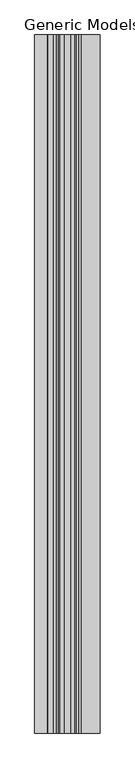
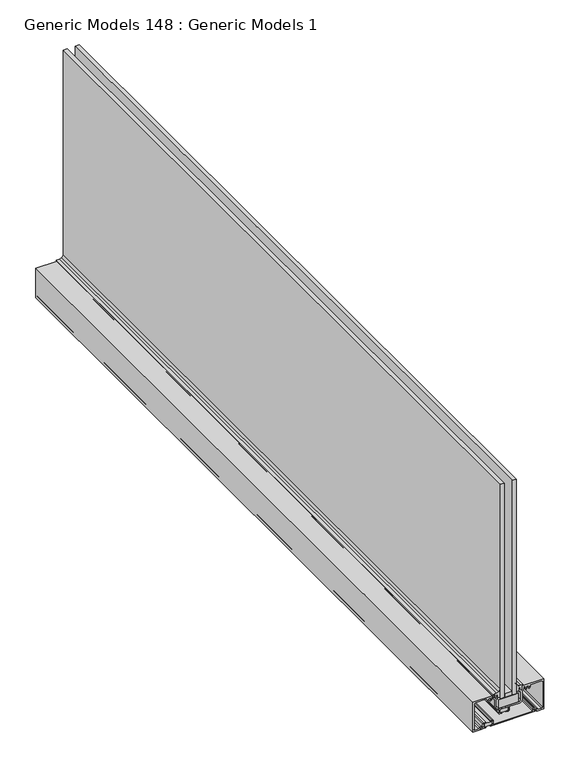
"""IFC4 building model written with IfcOpenShell, lengths in millimetres: proxy geometry, Generic Models 148 : Generic Models 1."""

from ifc_helpers import new_model, si_unit, point, frame, frame_2d, origin, place, context, project, spatial, polyline, circle_curve, trimmed, segment, composite_curve, outline, extrude, source, transform, mapped, element, save


def generic_models_148_generic_models_1_cbf84703(model_context):
    return source(origin(), model_context, "Body", "SweptSolid", [
        extrude(outline(composite_curve([segment(trimmed(circle_curve(frame_2d((-1910.3503206, 53784.0362451)), 1.5795625), [point((-1908.7707581, 53784.0362451))], [point((-1909.8092658, 53782.5522379))], False, "CARTESIAN"), True, "CONTINUOUS"), segment(polyline([(-1909.8092658, 53782.5522379), (-1913.6824831, 53781.1401001), (-1913.6824831, 53782.6297743), (-1916.2637581, 53782.6297743), (-1916.2637581, 53778.3117743), (-1917.8988831, 53778.3117743), (-1917.8988831, 53787.5924263), (-1916.2637581, 53787.5924263), (-1916.2637581, 53784.0110263), (-1909.6438831, 53784.0110263), (-1909.6438831, 53787.5924263), (-1908.7707581, 53787.5924263), (-1908.7707581, 53784.0362451)]), True, "CONTINUOUS")], self_intersect=False)), frame((0.0, 0.0, 0.0), z_axis=(0.0, 1.0, 0.0), x_axis=(0.0, 0.0, 1.0)), (0.0, 0.0, 1.0), 1219.2),
        extrude(outline(composite_curve([segment(trimmed(circle_curve(frame_2d((-1912.0013206, 53863.1457105)), 0.7064375), [point((-1911.7594231, 53863.809442))], [point((-1912.7064566, 53863.102848))], True, "CARTESIAN"), True, "CONTINUOUS"), segment(polyline([(-1912.7064566, 53863.102848), (-1916.2637581, 53863.102848), (-1916.2637581, 53800.0082638)]), True, "CONTINUOUS"), segment(trimmed(circle_curve(frame_2d((-1915.5573206, 53800.0082638)), 0.7064375), [point((-1916.2637581, 53800.0082638))], [point((-1915.5573206, 53799.3018263))], True, "CARTESIAN"), True, "CONTINUOUS"), segment(polyline([(-1915.5573206, 53799.3018263), (-1910.3503206, 53799.3018263)]), True, "CONTINUOUS"), segment(trimmed(circle_curve(frame_2d((-1910.3503206, 53797.7222638)), 1.5795625), [point((-1910.3503206, 53799.3018263))], [point((-1908.7707581, 53797.7222638))], False, "CARTESIAN"), True, "CONTINUOUS"), segment(polyline([(-1908.7707581, 53797.7222638), (-1908.7707581, 53794.3393013), (-1909.6438831, 53794.3393013), (-1909.6438831, 53797.9207013), (-1916.2637581, 53797.9207013), (-1916.2637581, 53794.3393013), (-1917.8988831, 53794.3393013), (-1917.8988831, 53868.801973), (-1916.2637581, 53868.801973), (-1916.2637581, 53864.483973), (-1913.6824831, 53864.483973), (-1913.6824831, 53865.9736472), (-1908.4373356, 53864.0613168)]), True, "CONTINUOUS"), segment(trimmed(circle_curve(frame_2d((-1908.6739206, 53863.4124105)), 0.6906895), [point((-1908.4373356, 53864.0613168))], [point((-1908.9099064, 53862.763286))], False, "CARTESIAN"), True, "CONTINUOUS"), segment(polyline([(-1908.9099064, 53862.763286), (-1911.7594231, 53863.809442)]), True, "CONTINUOUS")], self_intersect=False)), frame((0.0, 0.0, 0.0), z_axis=(0.0, 1.0, 0.0), x_axis=(0.0, 0.0, 1.0)), (0.0, 0.0, 1.0), 1219.2),
        extrude(outline(composite_curve([segment(trimmed(circle_curve(frame_2d((-1890.1573206, 53841.0696108)), 2.54), [point((-1890.1573206, 53843.6096108))], [point((-1892.6973206, 53841.0696108))], True, "CARTESIAN"), True, "CONTINUOUS"), segment(polyline([(-1892.6973206, 53841.0696108), (-1892.6973206, 53819.5939108), (-1894.7293206, 53819.5939108), (-1894.7293206, 53823.1753108), (-1900.9523206, 53823.1753108), (-1900.9523206, 53819.5939108), (-1902.2223206, 53819.5939108), (-1902.2223206, 53823.1753108)]), True, "CONTINUOUS"), segment(trimmed(circle_curve(frame_2d((-1900.4443206, 53823.1753108)), 1.778), [point((-1902.2223206, 53823.1753108))], [point((-1900.4443206, 53824.9533108))], False, "CARTESIAN"), True, "CONTINUOUS"), segment(polyline([(-1900.4443206, 53824.9533108), (-1895.2373206, 53824.9533108)]), True, "CONTINUOUS"), segment(trimmed(circle_curve(frame_2d((-1895.2373206, 53825.4613108)), 0.508), [point((-1895.2373206, 53824.9533108))], [point((-1894.7293206, 53825.4613108))], True, "CARTESIAN"), True, "CONTINUOUS"), segment(polyline([(-1894.7293206, 53825.4613108), (-1894.7293206, 53841.3236108)]), True, "CONTINUOUS"), segment(trimmed(circle_curve(frame_2d((-1890.4113206, 53841.3236108)), 4.318), [point((-1894.7293206, 53841.3236108))], [point((-1890.4113206, 53845.6416108))], False, "CARTESIAN"), True, "CONTINUOUS"), segment(polyline([(-1890.4113206, 53845.6416108), (-1875.313095, 53845.6416108), (-1873.608637, 53847.3474845)]), True, "CONTINUOUS"), segment(trimmed(circle_curve(frame_2d((-1871.7220005, 53845.4624138)), 2.667), [point((-1873.608637, 53847.3474845))], [point((-1871.7220005, 53848.1294138))], False, "CARTESIAN"), True, "CONTINUOUS"), segment(polyline([(-1871.7220005, 53848.1294138), (-1869.8373206, 53848.1294138)]), True, "CONTINUOUS"), segment(trimmed(circle_curve(frame_2d((-1869.8373206, 53848.6374138)), 0.508), [point((-1869.8373206, 53848.1294138))], [point((-1869.3293206, 53848.6374138))], True, "CARTESIAN"), True, "CONTINUOUS"), segment(polyline([(-1869.3293206, 53848.6374138), (-1869.3293206, 53850.4489459)]), True, "CONTINUOUS"), segment(trimmed(circle_curve(frame_2d((-1869.8373206, 53850.4489459)), 0.508), [point((-1869.3293206, 53850.4489459))], [point((-1870.0789638, 53850.8957933))], True, "CARTESIAN"), True, "CONTINUOUS"), segment(trimmed(circle_curve(frame_2d((-1872.0725206, 53854.5822838)), 4.191), [point((-1870.0789638, 53850.8957933))], [point((-1875.1205206, 53851.7057969))], False, "CARTESIAN"), True, "CONTINUOUS"), segment(polyline([(-1875.1205206, 53851.7057969), (-1875.1205206, 53852.8225202), (-1874.1622399, 53853.3757838)]), True, "CONTINUOUS"), segment(trimmed(circle_curve(frame_2d((-1872.0725206, 53854.5822838)), 2.413), [point((-1874.1622399, 53853.3757838))], [point((-1874.1622399, 53855.7887838))], True, "CARTESIAN"), True, "CONTINUOUS"), segment(polyline([(-1874.1622399, 53855.7887838), (-1875.1205206, 53856.3420474), (-1875.1205206, 53857.4587707)]), True, "CONTINUOUS"), segment(trimmed(circle_curve(frame_2d((-1872.0725206, 53854.5822838)), 4.191), [point((-1875.1205206, 53857.4587707))], [point((-1870.0789638, 53858.2687744))], False, "CARTESIAN"), True, "CONTINUOUS"), segment(trimmed(circle_curve(frame_2d((-1869.8373206, 53858.7156217)), 0.508), [point((-1870.0789638, 53858.2687744))], [point((-1869.3293206, 53858.7156217))], True, "CARTESIAN"), True, "CONTINUOUS"), segment(polyline([(-1869.3293206, 53858.7156217), (-1869.3293206, 53877.2009838)]), True, "CONTINUOUS"), segment(trimmed(circle_curve(frame_2d((-1870.8533206, 53877.2009838)), 1.524), [point((-1869.3293206, 53877.2009838))], [point((-1870.8533206, 53878.7249838))], True, "CARTESIAN"), True, "CONTINUOUS"), segment(polyline([(-1870.8533206, 53878.7249838), (-1914.5413206, 53878.7249838)]), True, "CONTINUOUS"), segment(trimmed(circle_curve(frame_2d((-1914.5413206, 53877.2009838)), 1.524), [point((-1914.5413206, 53878.7249838))], [point((-1916.0653206, 53877.2009838))], True, "CARTESIAN"), True, "CONTINUOUS"), segment(polyline([(-1916.0653206, 53877.2009838), (-1916.0653206, 53871.1448248)]), True, "CONTINUOUS"), segment(trimmed(circle_curve(frame_2d((-1915.5573206, 53869.7079838)), 1.524), [point((-1916.0653206, 53871.1448248))], [point((-1914.0333206, 53869.7079838))], False, "CARTESIAN"), True, "CONTINUOUS"), segment(polyline([(-1914.0333206, 53869.7079838), (-1914.0333206, 53864.9498123)]), True, "CONTINUOUS"), segment(trimmed(circle_curve(frame_2d((-1914.4905206, 53866.4567838)), 1.5748), [point((-1914.0333206, 53864.9498123))], [point((-1916.0653206, 53866.4567838))], False, "CARTESIAN"), True, "CONTINUOUS"), segment(polyline([(-1916.0653206, 53866.4567838), (-1916.0653206, 53869.1999838), (-1918.0973206, 53869.1999838), (-1918.0973206, 53880.7569838), (-1867.2973206, 53880.7569838), (-1867.2973206, 53846.0974138), (-1871.9851806, 53846.0974138), (-1873.8632206, 53844.2178138), (-1873.8632206, 53842.7437599), (-1870.8660206, 53842.0854838), (-1869.0880206, 53842.0854838), (-1869.0880206, 53841.0694838), (-1875.1332206, 53841.0694838), (-1875.1332206, 53843.1016108)]), True, "CONTINUOUS"), segment(trimmed(circle_curve(frame_2d((-1875.6412206, 53843.1016108)), 0.508), [point((-1875.1332206, 53843.1016108))], [point((-1875.6412206, 53843.6096108))], True, "CARTESIAN"), True, "CONTINUOUS"), segment(polyline([(-1875.6412206, 53843.6096108), (-1890.1573206, 53843.6096108)]), True, "CONTINUOUS")], self_intersect=False)), frame((0.0, 0.0, 0.0), z_axis=(0.0, 1.0, 0.0), x_axis=(0.0, 0.0, 1.0)), (0.0, 0.0, 1.0), 1219.2),
        extrude(outline(composite_curve([segment(trimmed(circle_curve(frame_2d((-1875.6412206, 53804.1124838)), 0.508), [point((-1875.6412206, 53803.6044838))], [point((-1875.1332206, 53804.1124838))], True, "CARTESIAN"), True, "CONTINUOUS"), segment(polyline([(-1875.1332206, 53804.1124838), (-1875.1332206, 53806.1446108), (-1869.0880206, 53806.1446108), (-1869.0880206, 53805.1286108), (-1870.8660206, 53805.1286108), (-1873.8632206, 53804.4703348), (-1873.8632206, 53802.9962808), (-1871.9851806, 53801.1166808), (-1867.2973206, 53801.1166808), (-1867.2973206, 53766.4571108), (-1918.0973206, 53766.4571108), (-1918.0973206, 53778.0141108), (-1916.0653206, 53778.0141108), (-1916.0653206, 53780.7573108)]), True, "CONTINUOUS"), segment(trimmed(circle_curve(frame_2d((-1914.4905206, 53780.7573108)), 1.5748), [point((-1916.0653206, 53780.7573108))], [point((-1914.0333206, 53782.2642823))], False, "CARTESIAN"), True, "CONTINUOUS"), segment(polyline([(-1914.0333206, 53782.2642823), (-1914.0333206, 53777.5061108)]), True, "CONTINUOUS"), segment(trimmed(circle_curve(frame_2d((-1915.5573206, 53777.5061108)), 1.524), [point((-1914.0333206, 53777.5061108))], [point((-1916.0653206, 53776.0692698))], False, "CARTESIAN"), True, "CONTINUOUS"), segment(polyline([(-1916.0653206, 53776.0692698), (-1916.0653206, 53770.0129838)]), True, "CONTINUOUS"), segment(trimmed(circle_curve(frame_2d((-1914.5413206, 53770.0129838)), 1.524), [point((-1916.0653206, 53770.0129838))], [point((-1914.5413206, 53768.4889838))], True, "CARTESIAN"), True, "CONTINUOUS"), segment(polyline([(-1914.5413206, 53768.4889838), (-1870.8533206, 53768.4889838)]), True, "CONTINUOUS"), segment(trimmed(circle_curve(frame_2d((-1870.8533206, 53770.0129838)), 1.524), [point((-1870.8533206, 53768.4889838))], [point((-1869.3293206, 53770.0129838))], True, "CARTESIAN"), True, "CONTINUOUS"), segment(polyline([(-1869.3293206, 53770.0129838), (-1869.3293206, 53788.4984729)]), True, "CONTINUOUS"), segment(trimmed(circle_curve(frame_2d((-1869.8373206, 53788.4984729)), 0.508), [point((-1869.3293206, 53788.4984729))], [point((-1870.0789638, 53788.9453203))], True, "CARTESIAN"), True, "CONTINUOUS"), segment(trimmed(circle_curve(frame_2d((-1872.0725206, 53792.6318108)), 4.191), [point((-1870.0789638, 53788.9453203))], [point((-1875.1205206, 53789.7553239))], False, "CARTESIAN"), True, "CONTINUOUS"), segment(polyline([(-1875.1205206, 53789.7553239), (-1875.1205206, 53790.8720472), (-1874.1622399, 53791.4253108)]), True, "CONTINUOUS"), segment(trimmed(circle_curve(frame_2d((-1872.0725206, 53792.6318108)), 2.413), [point((-1874.1622399, 53791.4253108))], [point((-1874.1622399, 53793.8383108))], True, "CARTESIAN"), True, "CONTINUOUS"), segment(polyline([(-1874.1622399, 53793.8383108), (-1875.1205206, 53794.3915744), (-1875.1205206, 53795.5082977)]), True, "CONTINUOUS"), segment(trimmed(circle_curve(frame_2d((-1872.0725206, 53792.6318108)), 4.191), [point((-1875.1205206, 53795.5082977))], [point((-1870.0789638, 53796.3183014))], False, "CARTESIAN"), True, "CONTINUOUS"), segment(trimmed(circle_curve(frame_2d((-1869.8373206, 53796.7651487)), 0.508), [point((-1870.0789638, 53796.3183014))], [point((-1869.3293206, 53796.7651487))], True, "CARTESIAN"), True, "CONTINUOUS"), segment(polyline([(-1869.3293206, 53796.7651487), (-1869.3293206, 53798.5766808)]), True, "CONTINUOUS"), segment(trimmed(circle_curve(frame_2d((-1869.8373206, 53798.5766808)), 0.508), [point((-1869.3293206, 53798.5766808))], [point((-1869.8373206, 53799.0846808))], True, "CARTESIAN"), True, "CONTINUOUS"), segment(polyline([(-1869.8373206, 53799.0846808), (-1871.7220005, 53799.0846808)]), True, "CONTINUOUS"), segment(trimmed(circle_curve(frame_2d((-1871.7220005, 53801.7516808)), 2.667), [point((-1871.7220005, 53799.0846808))], [point((-1873.608637, 53799.8666101))], False, "CARTESIAN"), True, "CONTINUOUS"), segment(polyline([(-1873.608637, 53799.8666101), (-1875.313095, 53801.5724838), (-1890.4113206, 53801.5724838)]), True, "CONTINUOUS"), segment(trimmed(circle_curve(frame_2d((-1890.4113206, 53805.8904838)), 4.318), [point((-1890.4113206, 53801.5724838))], [point((-1894.7293206, 53805.8904838))], False, "CARTESIAN"), True, "CONTINUOUS"), segment(polyline([(-1894.7293206, 53805.8904838), (-1894.7293206, 53807.8843838), (-1900.4443206, 53807.8843838)]), True, "CONTINUOUS"), segment(trimmed(circle_curve(frame_2d((-1900.4443206, 53809.6623838)), 1.778), [point((-1900.4443206, 53807.8843838))], [point((-1902.2223206, 53809.6623838))], False, "CARTESIAN"), True, "CONTINUOUS"), segment(polyline([(-1902.2223206, 53809.6623838), (-1902.2223206, 53813.2439108), (-1900.9523206, 53813.2439108), (-1900.9523206, 53809.6625108), (-1894.7293206, 53809.6625108), (-1894.7293206, 53813.2439108), (-1892.6973206, 53813.2439108), (-1892.6973206, 53806.1444838)]), True, "CONTINUOUS"), segment(trimmed(circle_curve(frame_2d((-1890.1573206, 53806.1444838)), 2.54), [point((-1892.6973206, 53806.1444838))], [point((-1890.1573206, 53803.6044838))], True, "CARTESIAN"), True, "CONTINUOUS"), segment(polyline([(-1890.1573206, 53803.6044838), (-1875.6412206, 53803.6044838)]), True, "CONTINUOUS")], self_intersect=False)), frame((0.0, 0.0, 0.0), z_axis=(0.0, 1.0, 0.0), x_axis=(0.0, 0.0, 1.0)), (0.0, 0.0, 1.0), 1219.2),
        extrude(outline(polyline([(53839.5075786, 0.0), (53808.1544536, 0.0), (53808.1544536, 1219.2), (53839.5075786, 1219.2), (53839.5075786, 0.0)])), frame((0.0, 0.0, -1891.8480905), z_axis=(0.0, 0.0, 1.0), x_axis=(1.0, 0.0, 0.0)), (0.0, 0.0, 1.0), 14.684375),
        extrude(outline(polyline([(53817.2682008, 0.0), (53810.9182008, 0.0), (53810.9182008, 1219.2), (53817.2682008, 1219.2), (53817.2682008, 0.0)])), frame((0.0, 0.0, -1876.8223206), z_axis=(0.0, 0.0, 1.0), x_axis=(1.0, 0.0, 0.0)), (0.0, 0.0, 1.0), 365.125),
        extrude(outline(polyline([(53836.3182008, 0.0), (53829.9682008, 0.0), (53829.9682008, 1219.2), (53836.3182008, 1219.2), (53836.3182008, 0.0)])), frame((0.0, 0.0, -1876.8223206), z_axis=(0.0, 0.0, 1.0), x_axis=(1.0, 0.0, 0.0)), (0.0, 0.0, 1.0), 365.125),
        extrude(outline(polyline([(53829.7697633, 0.0), (53817.4666383, 0.0), (53817.4666383, 1219.2), (53829.7697633, 1219.2), (53829.7697633, 0.0)])), frame((0.0, 0.0, -1876.8223206), z_axis=(0.0, 0.0, 1.0), x_axis=(1.0, 0.0, 0.0)), (0.0, 0.0, 1.0), 6.35),
        extrude(outline(composite_curve([segment(trimmed(circle_curve(frame_2d((-1860.2168324, 53842.5872853)), 4.9643345), [point((-1865.1395508, 53843.2287373))], [point((-1863.8157717, 53839.1678917))], True, "CARTESIAN"), True, "CONTINUOUS"), segment(polyline([(-1863.8157717, 53839.1678917), (-1860.8565052, 53836.6190179), (-1873.7679916, 53836.6190179), (-1873.7679916, 53840.6004679), (-1868.3168339, 53840.6004679), (-1868.3168339, 53842.339141), (-1870.2119053, 53842.339141), (-1873.212428, 53842.9981468), (-1873.212428, 53843.9887376), (-1871.5667754, 53845.6357571), (-1866.9131122, 53845.6357571), (-1866.9131122, 53847.4131024), (-1865.7607324, 53847.4131024)]), True, "CONTINUOUS"), segment(trimmed(circle_curve(frame_2d((-1877.1320429, 53843.5867064)), 11.9978335), [point((-1865.7607324, 53847.4131024))], [point((-1865.1395508, 53843.2287373))], False, "CARTESIAN"), True, "CONTINUOUS")], self_intersect=False)), frame((0.0, 0.0, 0.0), z_axis=(0.0, 1.0, 0.0), x_axis=(0.0, 0.0, 1.0)), (0.0, 0.0, 1.0), 1219.2),
        extrude(outline(composite_curve([segment(trimmed(circle_curve(frame_2d((-1877.1320429, 53803.5024473)), 11.9978335), [point((-1865.1395508, 53803.8604163))], [point((-1865.7607324, 53799.6760513))], False, "CARTESIAN"), True, "CONTINUOUS"), segment(polyline([(-1865.7607324, 53799.6760513), (-1866.9131122, 53799.6760513), (-1866.9131122, 53801.4533965), (-1871.5667754, 53801.4533965), (-1873.212428, 53803.100416), (-1873.212428, 53804.0910068), (-1870.2119053, 53804.7500127), (-1868.3168339, 53804.7500127), (-1868.3168339, 53806.4886857), (-1873.7679916, 53806.4886857), (-1873.7679916, 53810.4701357), (-1860.8565052, 53810.4701357), (-1863.8157717, 53807.921262)]), True, "CONTINUOUS"), segment(trimmed(circle_curve(frame_2d((-1860.2168324, 53804.5018684)), 4.9643345), [point((-1863.8157717, 53807.921262))], [point((-1865.1395508, 53803.8604163))], True, "CARTESIAN"), True, "CONTINUOUS")], self_intersect=False)), frame((0.0, 0.0, 0.0), z_axis=(0.0, 1.0, 0.0), x_axis=(0.0, 0.0, 1.0)), (0.0, 0.0, 1.0), 1219.2),
        extrude(outline(polyline([(53797.5238263, 0.0), (53784.4079013, 0.0), (53784.4079013, 1219.2), (53797.5238263, 1219.2), (53797.5238263, 0.0)])), frame((0.0, 0.0, -1915.8668831), z_axis=(0.0, 0.0, 1.0), x_axis=(1.0, 0.0, 0.0)), (0.0, 0.0, 1.0), 5.826125),
        extrude(outline(polyline([(53822.9768733, 0.0), (53809.8609483, 0.0), (53809.8609483, 1219.2), (53822.9768733, 1219.2), (53822.9768733, 0.0)])), frame((0.0, 0.0, -1900.7538831), z_axis=(0.0, 0.0, 1.0), x_axis=(1.0, 0.0, 0.0)), (0.0, 0.0, 1.0), 5.826125),
    ])


if __name__ == "__main__":
    model = new_model("IFC4")
    model_context = context("Model", 3, world=origin())
    ifc_project = project(units=[si_unit("LENGTHUNIT", "METRE", prefix="MILLI")], contexts=[model_context])
    site = spatial("IfcSite", under=ifc_project)
    building = spatial("IfcBuilding", under=site)
    placement = place(None, origin())
    generic_models_148_generic_models_1_shape = generic_models_148_generic_models_1_cbf84703(model_context)
    element("IfcBuildingElementProxy", 1, Name="Generic Models 148 : Generic Models 1", ObjectType="Generic Models 148 : Generic Models 1", at=placement, inside=building, context=model_context, shape_type="MappedRepresentation", body=[
        mapped(generic_models_148_generic_models_1_shape, transform((0.0, 0.0, 0.0), x_axis=(1.0, 0.0, 0.0), y_axis=(0.0, 1.0, 0.0), z_axis=(0.0, 0.0, 1.0))),
    ])
    save(model, "model.ifc")

# Revit data of these elements
# Element 1 (IfcBuildingElementProxy, "Generic Models 148 : Generic Models 1")
#   Materials on its faces: "ALUM. STOREFRONT W/ INSULATED GLAZING"
# Materials
#   "ALUM. STOREFRONT W/ INSULATED GLAZING": class "Glass", colour RGB 196 205 210, transparency 0.85, Description = "Soda Lime Glass", Cost = 0
